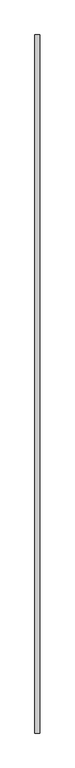
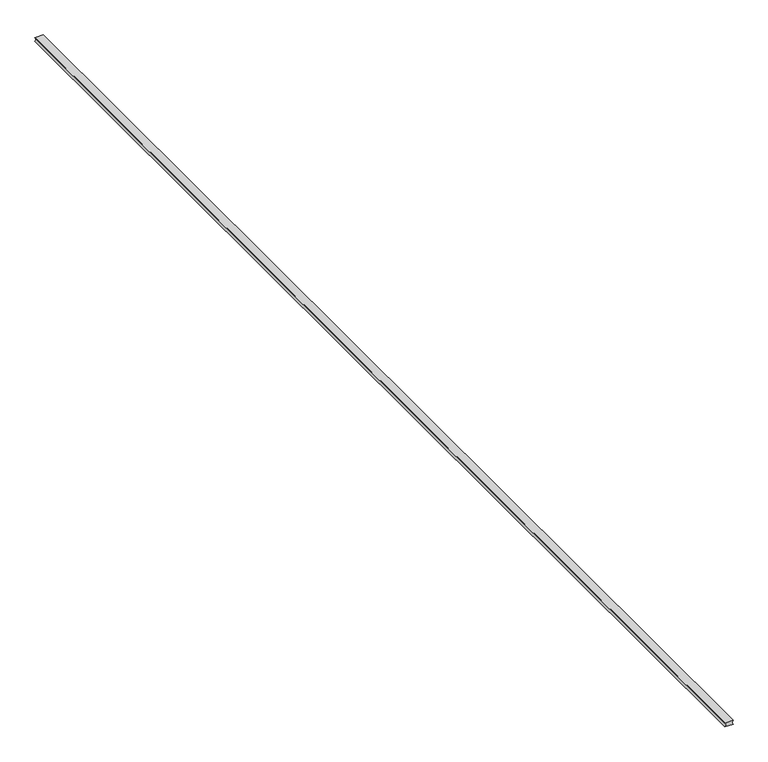
"""IFC4 building model written with IfcOpenShell, lengths in millimetres: proxy geometry, Joint039 5824 : Joint039 5824."""

from ifc_helpers import new_model, si_unit, point, frame, frame_2d, origin, place, context, project, spatial, polyline, circle_curve, trimmed, segment, composite_curve, outline, extrude, source, transform, mapped, element, save


def generic_models_7fa7a819(model_context):
    return source(origin(), model_context, "Body", "SweptSolid", [
        extrude(outline(composite_curve([segment(trimmed(circle_curve(frame_2d((40791.0390625, 16651.9501291)), 5.066659), [point((40787.71875, 16648.1230469))], [point((40794.359375, 16648.1230469))], True, "CARTESIAN"), True, "CONTINUOUS"), segment(polyline([(40794.359375, 16648.1230469), (40794.359375, 16634.4429202)]), True, "CONTINUOUS"), segment(trimmed(circle_curve(frame_2d((40791.0390625, 16630.6158379)), 5.066659), [point((40794.359375, 16634.4429202))], [point((40787.71875, 16634.4429202))], True, "CARTESIAN"), True, "CONTINUOUS"), segment(polyline([(40787.71875, 16634.4429202), (40787.71875, 16648.1230469)]), True, "CONTINUOUS")], self_intersect=False)), frame((0.0, 7982.1448924, 0.0), z_axis=(0.0, 1.0, 0.0), x_axis=(0.0, 0.0, 1.0)), (0.0, 0.0, 1.0), 2000.0),
    ])


if __name__ == "__main__":
    model = new_model("IFC4")
    model_context = context("Model", 3, world=origin())
    ifc_project = project(units=[si_unit("LENGTHUNIT", "METRE", prefix="MILLI")], contexts=[model_context])
    site = spatial("IfcSite", under=ifc_project)
    building = spatial("IfcBuilding", under=site)
    placement = place(None, origin())
    generic_models_shape = generic_models_7fa7a819(model_context)
    element("IfcBuildingElementProxy", 1, Name="Joint039 5824 : Joint039 5824", ObjectType="Joint039 5824 : Joint039 5824", at=placement, inside=building, context=model_context, shape_type="MappedRepresentation", body=[
        mapped(generic_models_shape, transform((0.0, 0.0, 0.0), x_axis=(1.0, 0.0, 0.0), y_axis=(0.0, 1.0, 0.0), z_axis=(0.0, 0.0, 1.0))),
    ])
    save(model, "model.ifc")

# Revit data of these elements
# Type "Joint039 5824 : Joint039 5824"
#   NameOverride = "Joint039"
# Element 1 (IfcBuildingElementProxy, "Joint039 5824 : Joint039 5824")
#   Materials on its faces: "SEALANT"
# Materials
#   "SEALANT": class "Unassigned", colour RGB 142 225 148, transparency 0
